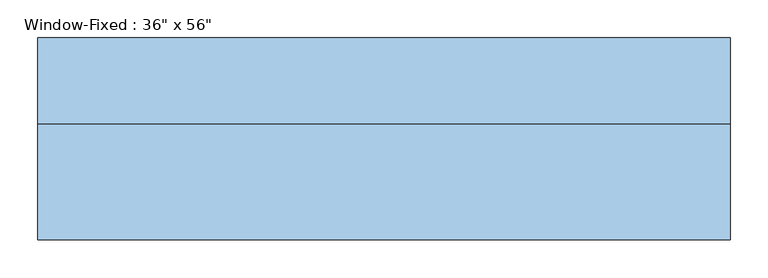
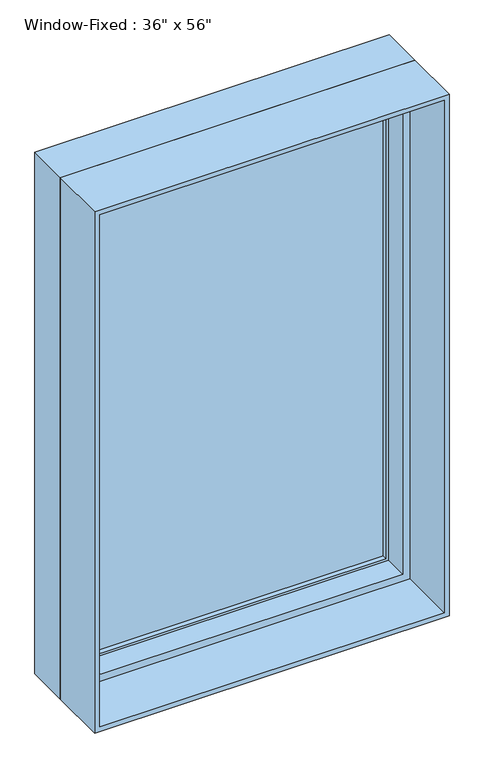
"""IFC4 building model written with IfcOpenShell, lengths in millimetres: window geometry."""

from ifc_helpers import new_model, si_unit, frame, origin, place, context, project, spatial, polyline, outline, extrude, faceted_brep, source, transform, mapped, element, save


def window_b51ec15c(model_context):
    return source(origin(), model_context, "Body", "SolidModel", [
        extrude(outline(polyline([(419.1, 79.375), (419.1, 73.025), (-419.1, 73.025), (-419.1, 79.375), (419.1, 79.375)])), frame((0.0, 0.0, 952.5), z_axis=(0.0, 0.0, 1.0), x_axis=(1.0, 0.0, 0.0)), (0.0, 0.0, 1.0), 1346.2),
        extrude(outline(polyline([(-419.1, 60.325), (-419.1, 66.675), (419.1, 66.675), (419.1, 60.325), (-419.1, 60.325)])), frame((0.0, 0.0, 952.5), z_axis=(0.0, 0.0, 1.0), x_axis=(1.0, 0.0, 0.0)), (0.0, 0.0, 1.0), 1346.2),
        extrude(outline(polyline([(927.1, 444.5), (2324.1, 444.5), (2324.1, -444.5), (927.1, -444.5), (927.1, 444.5)]), holes=[polyline([(952.5, -419.1), (2298.7, -419.1), (2298.7, 419.1), (952.5, 419.1), (952.5, -419.1)])]), frame((0.0, 47.625, 0.0), z_axis=(0.0, 1.0, 0.0), x_axis=(0.0, 0.0, 1.0)), (0.0, 0.0, 1.0), 44.45),
        extrude(outline(polyline([(2336.8, -457.2), (914.4, -457.2), (914.4, 457.2), (2336.8, 457.2), (2336.8, -457.2)]), holes=[polyline([(2324.1, 444.5), (927.1, 444.5), (927.1, -444.5), (2324.1, -444.5), (2324.1, 444.5)])]), frame((0.0, -168.275, 0.0), z_axis=(0.0, 1.0, 0.0), x_axis=(0.0, 0.0, 1.0)), (0.0, 0.0, 1.0), 152.4),
        faceted_brep([(457.2, -15.875, 2336.8), (457.2, 98.425, 2336.8), (-457.2, 98.425, 2336.8), (-457.2, -15.875, 2336.8), (-457.2, 98.425, 914.4), (-457.2, -15.875, 914.4), (457.2, 98.425, 914.4), (457.2, -15.875, 914.4), (425.45, -15.875, 2305.05), (425.45, -15.875, 946.15), (-425.45, -15.875, 946.15), (-425.45, -15.875, 2305.05), (-444.5, 98.425, 2324.1), (-444.5, 98.425, 927.1), (444.5, 98.425, 927.1), (444.5, 98.425, 2324.1), (425.45, 47.625, 2305.05), (-425.45, 47.625, 2305.05), (444.5, 47.625, 2324.1), (-444.5, 47.625, 2324.1), (-425.45, 47.625, 946.15), (-444.5, 47.625, 927.1), (425.45, 47.625, 946.15), (444.5, 47.625, 927.1)], [[[0, 1, 2, 3]], [[3, 2, 4, 5]], [[5, 4, 6, 7]], [[3, 5, 7, 0], [8, 9, 10, 11]], [[7, 6, 1, 0]], [[1, 6, 4, 2], [12, 13, 14, 15]], [[16, 8, 11, 17]], [[15, 18, 19, 12]], [[17, 11, 10, 20]], [[12, 19, 21, 13]], [[20, 10, 9, 22]], [[13, 21, 23, 14]], [[22, 9, 8, 16]], [[18, 23, 21, 19], [17, 20, 22, 16]], [[14, 23, 18, 15]]]),
    ])


if __name__ == "__main__":
    model = new_model("IFC4")
    model_context = context("Model", 3, world=origin())
    ifc_project = project(units=[si_unit("LENGTHUNIT", "METRE", prefix="MILLI")], contexts=[model_context])
    site = spatial("IfcSite", under=ifc_project)
    building = spatial("IfcBuilding", under=site)
    placement = place(None, origin())
    window_shape = window_b51ec15c(model_context)
    element("IfcWindow", 1, ObjectType="Window-Fixed : 36\" x 56\"", at=placement, inside=building, context=model_context, shape_type="MappedRepresentation", body=[
        mapped(window_shape, transform((0.0, 0.0, 0.0), x_axis=(1.0, 0.0, 0.0), y_axis=(0.0, 1.0, 0.0), z_axis=(0.0, 0.0, 1.0))),
    ])
    save(model, "model.ifc")

# Revit data of these elements
# Type "Window-Fixed : 36\" x 56\""
#   Type Mark = "22"
#   Fire Rating = "0.5h"
#   Assembly Code = "B2020100"
#   Analytic Construction = "Double glazing - domestic"
#   Window Inset [instance default] = 0' - 0"
#   Wall Thickness [instance default] = 0' - 6"
#   Visual Light Transmittance = 0.81
#   Thermal Resistance (R) = 1.8146 (h·ft²·°F)/BTU
#   Solar Heat Gain Coefficient = 0.76
#   Rough Width = 3' - 0 1/2"
#   Rough Height = 4' - 8 1/2"
#   Interior Wall Closure [instance default] = 0' - 2 1/4"
#   Height = 4' - 8"
#   Heat Transfer Coefficient (U) = 0.5511 BTU/(h·ft²·°F)
#   Frame Extension [instance default] = 0' - 0 1/4"
#   Exterior Wall Closure [instance default] = 0' - 1 1/4"
#   Extension Jamb [instance default] = 0' - 2 1/4"
#   Default Sill Height = 3' - 0"
#   Width = 3' - 0"
#   Muntin Visibility = yes
#   Interior Trim Visibility [instance default] = yes
#   Exterior Trim Visibility [instance default] = yes
#   Extension Jamb Visibility [instance default] = yes
#   Muntin Pattern = Muntin Pattern_2x2 : Muntin Pattern_2x2
#   Interior Trim Material = Wood - Stained
#   Interior Trim = Trim-Window-Interior-Flat : Picture Frame
#   Interior Frame Material = Wood - Stained
#   Glass Panel Material = Glass
#   Exterior Trim Material = Clad - White
#   Exterior Trim = Trim-Window-Exterior-Flat : with Sill
#   Exterior Frame Material = Clad - White
#   Wall Closure = (empty or 0)
# Element 1 (IfcWindow, "Window-Fixed : 36\" x 56\"")
#   Window Inset = 0' - 3 1/2"
#   Wall Thickness = 1' - 1 1/4"
#   Exterior Wall Closure = 0' - 5 1/2"
#   Extension Jamb = 0' - 6"
#   Exterior Trim Visibility = no
#   Materials on its faces: "Wood - Stained", "Glass", "Clad - White"
# Materials
#   "Wood - Stained": class "Wood", colour RGB 224 178 126, transparency 0, Cost = 0
#   "Glass": class "Glass", colour RGB 0 128 192, transparency 0.75, Description = "Soda Lime Glass", Cost = 0
#   "Clad - White": class "Wood", colour RGB 242 242 238, transparency 0, Cost = 0
